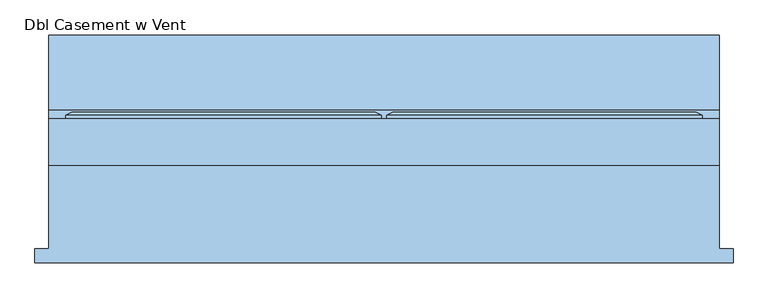
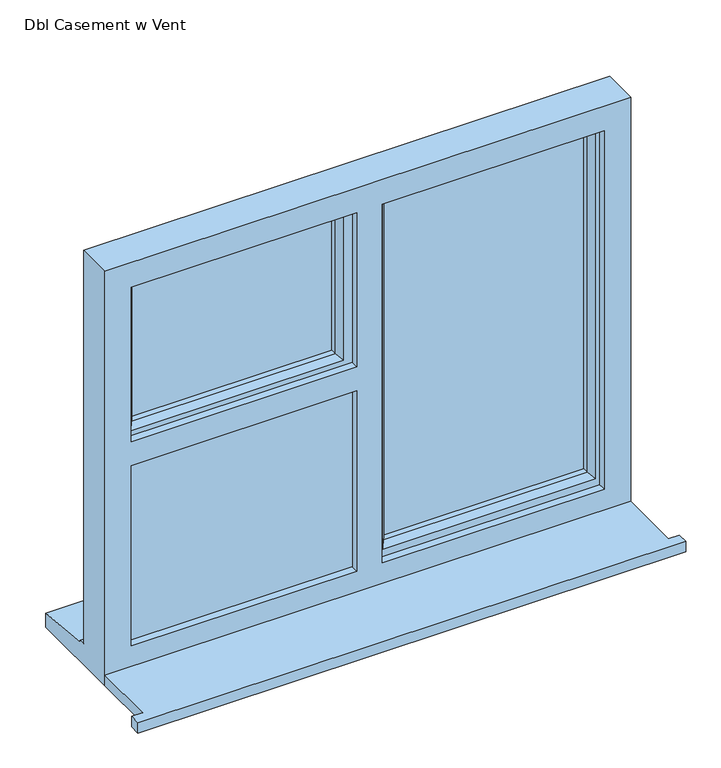
"""IFC4 building model written with IfcOpenShell, lengths in millimetres: window geometry, Dbl Casement w Vent : Doublel Casement with Vent 1200w x 1000h."""

from ifc_helpers import new_model, si_unit, frame, origin, place, context, project, spatial, polyline, outline, extrude, faceted_brep, source, transform, mapped, element, save


def dbl_casement_w_vent_67fd5172(model_context):
    return source(origin(), model_context, "Body", "SolidModel", [
        extrude(outline(polyline([(-910.0, -182.7934322), (-910.0, -157.7934322), (-885.0, -157.7934322), (-885.0, -8.2934322), (315.0, -8.2934322), (315.0, -157.7934322), (340.0, -157.7934322), (340.0, -182.7934322), (-910.0, -182.7934322)])), frame((0.0, 0.0, 1110.0), z_axis=(0.0, 0.0, 1.0), x_axis=(1.0, 0.0, 0.0)), (0.0, 0.0, 1.0), 25.0),
        faceted_brep([(-855.0, 74.7065678, 2080.0), (-855.0, 80.4800705, 2080.0), (-855.0, 80.4800705, 1650.0), (-855.0, 74.7065678, 1650.0), (-845.0, 9.7065678, 2070.0), (-845.0, 74.7065678, 2070.0), (-845.0, 74.7065678, 1660.0), (-845.0, 9.7065678, 1660.0), (-805.0, 24.1994677, 2030.0), (-815.1480377, 9.7065678, 2040.1480377), (-815.1480377, 9.7065678, 1689.8519623), (-805.0, 24.1994677, 1700.0), (-805.0, 38.7065678, 2030.0), (-805.0, 38.7065678, 1700.0), (-815.0, 62.7065678, 2040.0), (-815.0, 38.7065678, 2040.0), (-815.0, 38.7065678, 1690.0), (-815.0, 62.7065678, 1690.0), (-805.0, 80.4800705, 2030.0), (-805.0, 62.7065678, 2030.0), (-805.0, 62.7065678, 1700.0), (-805.0, 80.4800705, 1700.0), (-822.4457548, 86.2535732, 2047.4457548), (-822.4457548, 86.2535732, 1682.5542452), (-844.2153903, 86.2535732, 2069.2153903), (-844.2153903, 86.2535732, 1660.7846097), (-290.0, 80.4800705, 1650.0), (-290.0, 74.7065678, 1650.0), (-300.0, 74.7065678, 1660.0), (-300.0, 9.7065678, 1660.0), (-329.8519623, 9.7065678, 1689.8519623), (-340.0, 24.1994677, 1700.0), (-340.0, 38.7065678, 1700.0), (-330.0, 38.7065678, 1690.0), (-330.0, 62.7065678, 1690.0), (-340.0, 62.7065678, 1700.0), (-340.0, 80.4800705, 1700.0), (-322.5542452, 86.2535732, 1682.5542452), (-300.7846097, 86.2535732, 1660.7846097), (-290.0, 80.4800705, 2080.0), (-290.0, 74.7065678, 2080.0), (-300.0, 74.7065678, 2070.0), (-300.0, 9.7065678, 2070.0), (-329.8519623, 9.7065678, 2040.1480377), (-340.0, 24.1994677, 2030.0), (-340.0, 38.7065678, 2030.0), (-330.0, 38.7065678, 2040.0), (-330.0, 62.7065678, 2040.0), (-340.0, 62.7065678, 2030.0), (-340.0, 80.4800705, 2030.0), (-322.5542452, 86.2535732, 2047.4457548), (-300.7846097, 86.2535732, 2069.2153903)], [[[0, 1, 2, 3]], [[4, 5, 6, 7]], [[8, 9, 10, 11]], [[12, 8, 11, 13]], [[14, 15, 16, 17]], [[18, 19, 20, 21]], [[22, 18, 21, 23]], [[1, 24, 25, 2]], [[3, 2, 26, 27]], [[7, 6, 28, 29]], [[11, 10, 30, 31]], [[13, 11, 31, 32]], [[17, 16, 33, 34]], [[21, 20, 35, 36]], [[23, 21, 36, 37]], [[2, 25, 38, 26]], [[27, 26, 39, 40]], [[29, 28, 41, 42]], [[31, 30, 43, 44]], [[32, 31, 44, 45]], [[34, 33, 46, 47]], [[36, 35, 48, 49]], [[37, 36, 49, 50]], [[26, 38, 51, 39]], [[40, 39, 1, 0]], [[3, 27, 40, 0], [5, 41, 28, 6]], [[42, 41, 5, 4]], [[7, 29, 42, 4], [9, 43, 30, 10]], [[44, 43, 9, 8]], [[45, 44, 8, 12]], [[15, 46, 33, 16], [13, 32, 45, 12]], [[47, 46, 15, 14]], [[17, 34, 47, 14], [19, 48, 35, 20]], [[49, 48, 19, 18]], [[50, 49, 18, 22]], [[24, 51, 38, 25], [23, 37, 50, 22]], [[39, 51, 24, 1]]]),
        extrude(outline(polyline([(245.0, 38.7065678), (-240.0, 38.7065678), (-240.0, 62.7065678), (245.0, 62.7065678), (245.0, 38.7065678)])), frame((0.0, 0.0, 1203.0), z_axis=(0.0, 0.0, 1.0), x_axis=(1.0, 0.0, 0.0)), (0.0, 0.0, 1.0), 837.0),
        extrude(outline(polyline([(-330.0, 38.7065678), (-815.0, 38.7065678), (-815.0, 62.7065678), (-330.0, 62.7065678), (-330.0, 38.7065678)])), frame((0.0, 0.0, 1690.0), z_axis=(0.0, 0.0, 1.0), x_axis=(1.0, 0.0, 0.0)), (0.0, 0.0, 1.0), 350.0),
        extrude(outline(polyline([(-845.0, 33.7065678), (-300.0, 33.7065678), (-300.0, 9.7065678), (-845.0, 9.7065678), (-845.0, 33.7065678)])), frame((0.0, 0.0, 1173.0), z_axis=(0.0, 0.0, 1.0), x_axis=(1.0, 0.0, 0.0)), (0.0, 0.0, 1.0), 457.0),
        faceted_brep([(315.0, -8.2934322, 2110.0), (-885.0, -8.2934322, 2110.0), (-885.0, -8.2934322, 1110.0), (315.0, -8.2934322, 1110.0), (-825.0, -8.2934322, 1185.0), (-825.0, -8.2934322, 1620.0), (-310.0, -8.2934322, 1620.0), (-310.0, -8.2934322, 1185.0), (-825.0, -8.2934322, 2050.0), (-310.0, -8.2934322, 2050.0), (-310.0, -8.2934322, 1678.0), (-825.0, -8.2934322, 1678.0), (-252.0, -8.2934322, 2050.0), (255.0, -8.2934322, 2050.0), (255.0, -8.2934322, 1185.0), (-252.0, -8.2934322, 1185.0), (-885.0, 74.7065678, 2110.0), (-885.0, 74.7065678, 1161.0), (-885.0, 89.7065678, 1159.68767), (-885.0, 89.7065678, 1154.7449676), (-885.0, 224.7065678, 1143.8088847), (-885.0, 224.7065678, 1110.0), (315.0, 74.7065678, 2110.0), (315.0, 74.7065678, 1161.0), (-310.0, 74.7065678, 1173.0), (-310.0, 74.7065678, 1620.0), (-845.0, 74.7065678, 1620.0), (-845.0, 74.7065678, 1173.0), (-310.0, 74.7065678, 2070.0), (-845.0, 74.7065678, 2070.0), (-845.0, 74.7065678, 1660.0), (-310.0, 74.7065678, 1660.0), (275.0, 74.7065678, 1173.0), (275.0, 74.7065678, 2070.0), (-270.0, 74.7065678, 2070.0), (-270.0, 74.7065678, 1173.0), (-845.0, 9.7065678, 2070.0), (-845.0, 9.7065678, 1660.0), (-845.0, 9.7065678, 1630.0), (-845.0, 9.7065678, 1173.0), (-845.0, 33.7065678, 1620.0), (-845.0, 33.7065678, 1630.0), (-300.0, 9.7065678, 2070.0), (-300.0, 9.7065678, 1660.0), (-310.0, 9.7065678, 2050.0), (-825.0, 9.7065678, 2050.0), (-825.0, 9.7065678, 1678.0), (-310.0, 9.7065678, 1678.0), (-270.0, 9.7065678, 2070.0), (275.0, 9.7065678, 2070.0), (275.0, 9.7065678, 1173.0), (-270.0, 9.7065678, 1173.0), (255.0, 9.7065678, 2050.0), (-252.0, 9.7065678, 2050.0), (-252.0, 9.7065678, 1185.0), (255.0, 9.7065678, 1185.0), (-300.0, 9.7065678, 1173.0), (-300.0, 9.7065678, 1630.0), (-825.0, 9.7065678, 1185.0), (-310.0, 9.7065678, 1185.0), (-310.0, 9.7065678, 1620.0), (-825.0, 9.7065678, 1620.0), (-310.0, 33.7065678, 2070.0), (-300.0, 33.7065678, 2070.0), (315.0, 224.7065678, 1110.0), (315.0, 224.7065678, 1143.8088847), (315.0, 89.7065678, 1154.7449676), (315.0, 89.7065678, 1159.68767), (-300.0, 33.7065678, 1660.0), (-300.0, 33.7065678, 1630.0), (-300.0, 33.7065678, 1173.0), (-310.0, 33.7065678, 1660.0), (-310.0, 33.7065678, 1173.0), (-310.0, 33.7065678, 1620.0)], [[[0, 1, 2, 3], [4, 5, 6, 7], [8, 9, 10, 11], [12, 13, 14, 15]], [[1, 16, 17, 18, 19, 20, 21, 2]], [[16, 22, 23, 17], [24, 25, 26, 27], [28, 29, 30, 31], [32, 33, 34, 35]], [[29, 36, 37, 30]], [[38, 39, 27, 26, 40, 41]], [[36, 42, 43, 37], [44, 45, 46, 47]], [[48, 49, 50, 51], [52, 53, 54, 55]], [[56, 39, 38, 57], [58, 59, 60, 61]], [[45, 8, 11, 46]], [[4, 58, 61, 5]], [[1, 0, 22, 16]], [[36, 29, 28, 62, 63, 42]], [[33, 49, 48, 34]], [[8, 45, 44, 9]], [[52, 13, 12, 53]], [[22, 0, 3, 64, 65, 66, 67, 23]], [[33, 32, 50, 49]], [[13, 52, 55, 14]], [[43, 42, 63, 68]], [[69, 70, 56, 57]], [[63, 62, 71, 68]], [[72, 70, 69, 41, 40, 73]], [[62, 28, 31, 71]], [[24, 72, 73, 25]], [[35, 34, 48, 51]], [[53, 12, 15, 54]], [[9, 44, 47, 10]], [[59, 7, 6, 60]], [[64, 3, 2, 21]], [[65, 64, 21, 20]], [[66, 65, 20, 19]], [[67, 66, 19, 18]], [[23, 67, 18, 17]], [[24, 27, 39, 56, 70, 72]], [[32, 35, 51, 50]], [[15, 14, 55, 54]], [[59, 58, 4, 7]], [[57, 38, 41, 69]], [[26, 25, 73, 40]], [[31, 30, 37, 43, 68, 71]], [[47, 46, 11, 10]], [[61, 60, 6, 5]]]),
        extrude(outline(polyline([(1660.0, -825.0), (1660.0, -845.0), (1173.0, -845.0), (1173.0, -310.0), (1193.0, -310.0), (1193.0, -825.0), (1660.0, -825.0)])), frame((0.0, 33.7065678, 0.0), z_axis=(0.0, 1.0, 0.0), x_axis=(0.0, 0.0, 1.0)), (0.0, 0.0, 1.0), 41.0),
        faceted_brep([(-280.0, 74.7065678, 2080.0), (-280.0, 80.4800705, 2080.0), (-280.0, 80.4800705, 1163.0), (-280.0, 74.7065678, 1163.0), (-270.0, 9.7065678, 2070.0), (-270.0, 74.7065678, 2070.0), (-270.0, 74.7065678, 1173.0), (-270.0, 9.7065678, 1173.0), (-230.0, 24.1994677, 2030.0), (-240.1480377, 9.7065678, 2040.1480377), (-240.1480377, 9.7065678, 1202.8519623), (-230.0, 24.1994677, 1213.0), (-230.0, 38.7065678, 2030.0), (-230.0, 38.7065678, 1213.0), (-240.0, 62.7065678, 2040.0), (-240.0, 38.7065678, 2040.0), (-240.0, 38.7065678, 1203.0), (-240.0, 62.7065678, 1203.0), (-230.0, 80.4800705, 2030.0), (-230.0, 62.7065678, 2030.0), (-230.0, 62.7065678, 1213.0), (-230.0, 80.4800705, 1213.0), (-247.4457548, 86.2535732, 2047.4457548), (-247.4457548, 86.2535732, 1195.5542452), (-269.2153903, 86.2535732, 2069.2153903), (-269.2153903, 86.2535732, 1173.7846097), (285.0, 80.4800705, 1163.0), (285.0, 74.7065678, 1163.0), (275.0, 74.7065678, 1173.0), (275.0, 9.7065678, 1173.0), (245.1480377, 9.7065678, 1202.8519623), (235.0, 24.1994677, 1213.0), (235.0, 38.7065678, 1213.0), (245.0, 38.7065678, 1203.0), (245.0, 62.7065678, 1203.0), (235.0, 62.7065678, 1213.0), (235.0, 80.4800705, 1213.0), (252.4457548, 86.2535732, 1195.5542452), (274.2153903, 86.2535732, 1173.7846097), (285.0, 80.4800705, 2080.0), (285.0, 74.7065678, 2080.0), (275.0, 74.7065678, 2070.0), (275.0, 9.7065678, 2070.0), (245.1480377, 9.7065678, 2040.1480377), (235.0, 24.1994677, 2030.0), (235.0, 38.7065678, 2030.0), (245.0, 38.7065678, 2040.0), (245.0, 62.7065678, 2040.0), (235.0, 62.7065678, 2030.0), (235.0, 80.4800705, 2030.0), (252.4457548, 86.2535732, 2047.4457548), (274.2153903, 86.2535732, 2069.2153903)], [[[0, 1, 2, 3]], [[4, 5, 6, 7]], [[8, 9, 10, 11]], [[12, 8, 11, 13]], [[14, 15, 16, 17]], [[18, 19, 20, 21]], [[22, 18, 21, 23]], [[1, 24, 25, 2]], [[3, 2, 26, 27]], [[7, 6, 28, 29]], [[11, 10, 30, 31]], [[13, 11, 31, 32]], [[17, 16, 33, 34]], [[21, 20, 35, 36]], [[23, 21, 36, 37]], [[2, 25, 38, 26]], [[27, 26, 39, 40]], [[29, 28, 41, 42]], [[31, 30, 43, 44]], [[32, 31, 44, 45]], [[34, 33, 46, 47]], [[36, 35, 48, 49]], [[37, 36, 49, 50]], [[26, 38, 51, 39]], [[40, 39, 1, 0]], [[3, 27, 40, 0], [5, 41, 28, 6]], [[42, 41, 5, 4]], [[7, 29, 42, 4], [9, 43, 30, 10]], [[44, 43, 9, 8]], [[45, 44, 8, 12]], [[15, 46, 33, 16], [13, 32, 45, 12]], [[47, 46, 15, 14]], [[17, 34, 47, 14], [19, 48, 35, 20]], [[49, 48, 19, 18]], [[50, 49, 18, 22]], [[24, 51, 38, 25], [23, 37, 50, 22]], [[39, 51, 24, 1]]]),
    ])


if __name__ == "__main__":
    model = new_model("IFC4")
    model_context = context("Model", 3, world=origin())
    ifc_project = project(units=[si_unit("LENGTHUNIT", "METRE", prefix="MILLI")], contexts=[model_context])
    site = spatial("IfcSite", under=ifc_project)
    building = spatial("IfcBuilding", under=site)
    placement = place(None, origin())
    dbl_casement_w_vent_shape = dbl_casement_w_vent_67fd5172(model_context)
    element("IfcWindow", 1, ObjectType="Dbl Casement w Vent : Doublel Casement with Vent 1200w x 1000h", at=placement, inside=building, context=model_context, shape_type="MappedRepresentation", body=[
        mapped(dbl_casement_w_vent_shape, transform((0.0, 0.0, 0.0), x_axis=(1.0, 0.0, 0.0), y_axis=(0.0, 1.0, 0.0), z_axis=(0.0, 0.0, 1.0))),
    ])
    save(model, "model.ifc")

# Revit data of these elements
# Type "Dbl Casement w Vent : Doublel Casement with Vent 1200w x 1000h"
#   Description = "Double Casement Window with Opening Sash Vents"
#   Type Mark = "45"
#   Operation = "TriplePanelRight"
#   Construction Type Id = "GSP4R"
#   Manufacturer = "Revit"
#   Keynote = "L10"
#   Analytic Construction = "1/8 in Pilkington single glazing"
#   Wrap Layers (Ext) from Ext = 102.5 mm
#   Wrap Layers (Int) from Ext = 177.5 mm
#   Window Board Projection = 25 mm
#   Window Board Extension = 25 mm
#   Visual Light Transmittance = 0.9
#   Vent Depth = 450 mm
#   Thermal Resistance (R) = 0.271106 (m²·K)/W
#   Solar Heat Gain Coefficient = 0.78
#   Rough Width = 1200 mm
#   Rough Height = 1000 mm
#   Frame Height = 1350 mm
#   Height = 1000 mm
#   Width = 1200 mm
#   Heat Transfer Coefficient (U) = 3.6886 W/(m²·K)
#   Glazing Thickness = 24 mm
#   FrameOffset - External = 100 mm
#   Frame Depth = 65 mm
#   Default Head Height = 2110 mm
#   Cill Depth = 150 mm
#   Cavity Closer Width = 75 mm
#   Cavity Closer Offset from Ext = 110 mm
#   Cavity Closer Depth = 105 mm
#   Vis - Cavity Closers = yes
#   Material Trim = Window Frame
#   Material Glass = Glass
#   Material Frame = Window Frame
#   Wall Closure = (empty or 0)
# Element 1 (IfcWindow, "Dbl Casement w Vent : Doublel Casement with Vent 1200w x 1000h")
#   Materials on its faces: "Window Frame", "Glass"
# Materials
#   "Window Frame": class "Miscellaneous", colour RGB 249 249 249, transparency 0, Keynote = "L10"
#   "Glass": class "Glass", colour RGB 0 128 192, transparency 0.9, Description = "Soda Lime Glass", Cost = 0
